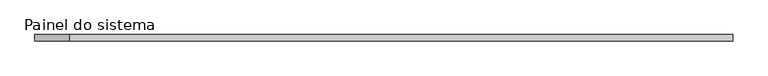
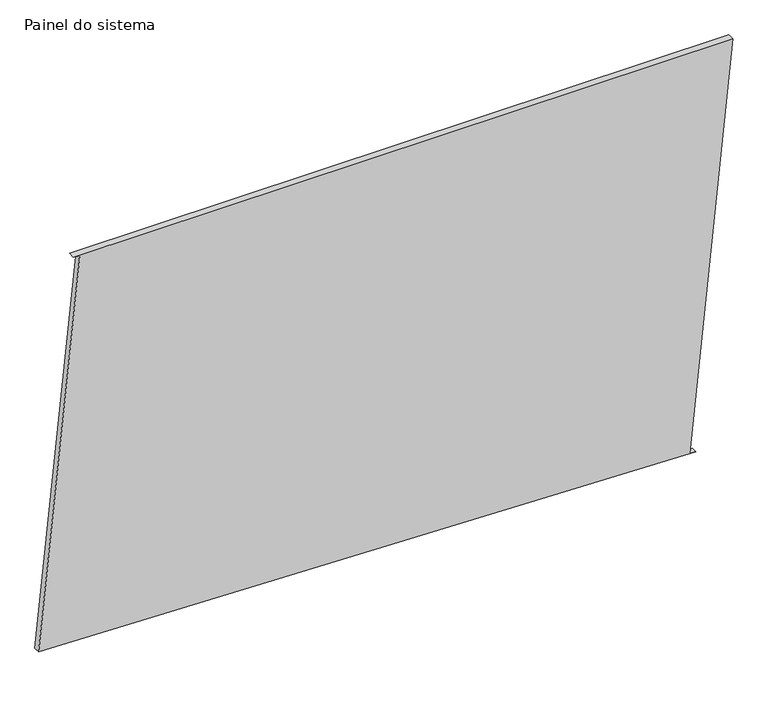
"""IFC4 building model written with IfcOpenShell, lengths in millimetres: plate geometry, Painel do sistema : Envidraçado."""

from ifc_helpers import new_model, si_unit, frame, origin, place, context, project, spatial, polyline, outline, extrude, source, transform, mapped, element, save


def painel_do_sistema_3904acbe(model_context):
    return source(origin(), model_context, "Body", "SweptSolid", [
        extrude(outline(polyline([(0.0, 1205.4838812), (2.5300763, 1180.6122364), (1646.4711205, 1347.8426832), (1646.4711205, -1212.9338164), (1643.9410442, -1188.0621717), (73.2357927, -1347.8426832), (0.0, 1205.4838812)])), frame((0.0, 24.5, 0.0), z_axis=(0.0, 1.0, 0.0), x_axis=(0.0, 0.0, 1.0)), (0.0, 0.0, 1.0), 25.0),
    ])


if __name__ == "__main__":
    model = new_model("IFC4")
    model_context = context("Model", 3, world=origin())
    ifc_project = project(units=[si_unit("LENGTHUNIT", "METRE", prefix="MILLI")], contexts=[model_context])
    site = spatial("IfcSite", under=ifc_project)
    building = spatial("IfcBuilding", under=site)
    placement = place(None, origin())
    painel_do_sistema_shape = painel_do_sistema_3904acbe(model_context)
    element("IfcPlate", 1, ObjectType="Painel do sistema : Envidraçado", at=placement, inside=building, context=model_context, shape_type="MappedRepresentation", body=[
        mapped(painel_do_sistema_shape, transform((0.0, 0.0, 0.0), x_axis=(1.0, 0.0, 0.0), y_axis=(0.0, 1.0, 0.0), z_axis=(0.0, 0.0, 1.0))),
    ])
    save(model, "model.ifc")

# Revit data of these elements
# Type "Painel do sistema : Envidraçado"
#   Construction Type Id = "GSP4R"
#   Analytic Construction = "Vidraça única Pilkington 1/8 pol"
#   Visual Light Transmittance = 0.9
#   Solar Heat Gain Coefficient = 0.86
#   Heat Transfer Coefficient (U) = 6.7069 W/(m²·K)
# Element 1 (IfcPlate, "Painel do sistema : Envidraçado")
#   Materials on its faces: "Vidro"
# Materials
#   "Vidro": class "Vidro", colour RGB 0 128 192, transparency 0.9, Description = "Vidro de sílica", Cost = 0
